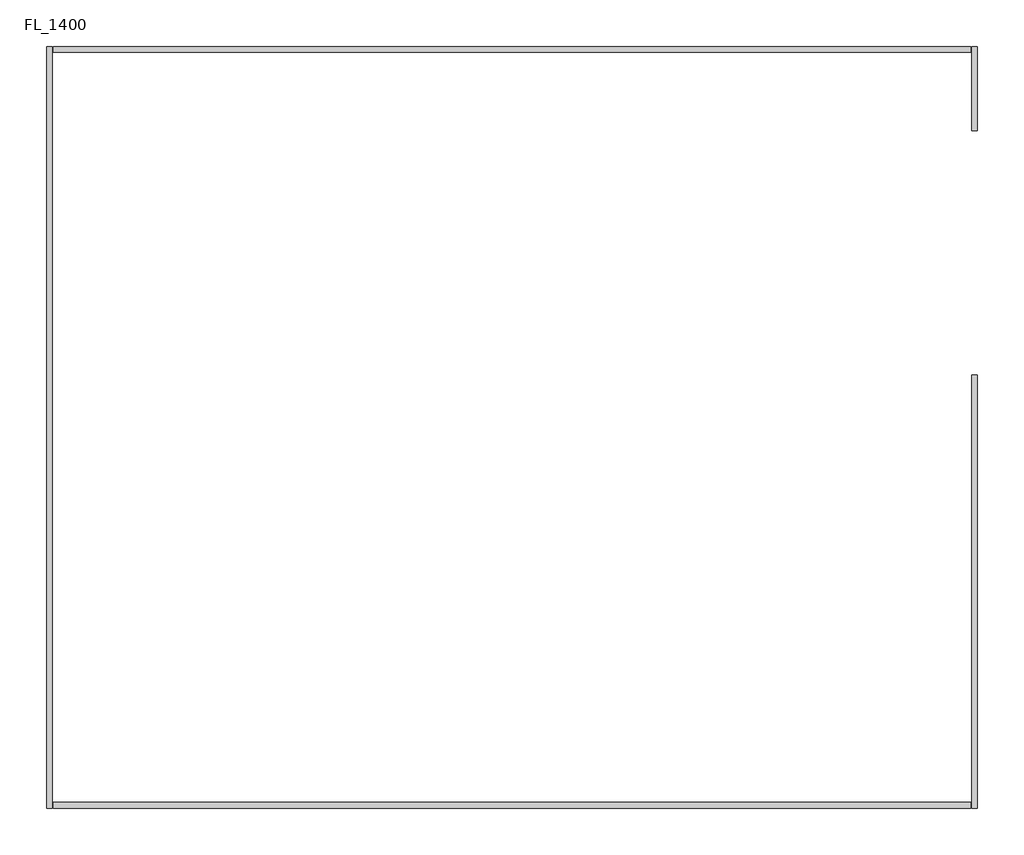
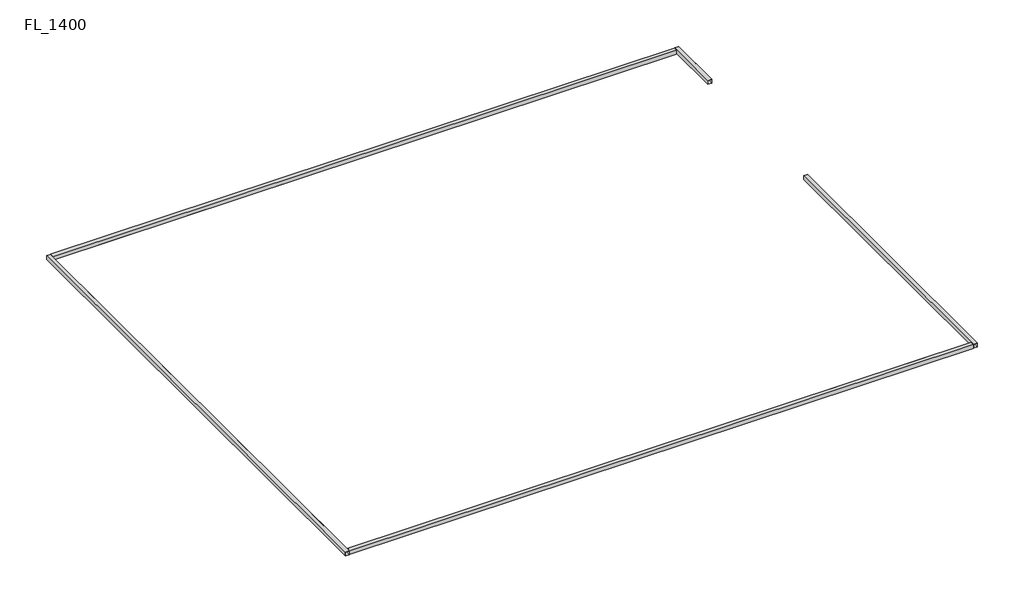
# One storey: 5 beams.
"""IFC4 building model written with IfcOpenShell, lengths in millimetres."""

import ifcopenshell
import ifcopenshell.guid

model = None  # the IFC model being written
_history = None  # IfcOwnerHistory: only IFC2X3 demands one
_inside = {}  # id of a spatial element -> (the spatial element, [elements in it])
_under = {}  # id of a project, library or spatial element -> (it, [spatial elements below it])
_declared = {}  # id of a project -> (the project, [libraries it declares])
_typed = {}  # id of a type object -> (the type object, [elements of that type])
_made_of = {}  # id of a material, layer set ... -> (it, [elements and type objects made of it])


def new_model(schema):
    """Start an empty IFC model of exactly this schema.

    Asked for "IFC4X3", IfcOpenShell would pick the latest addendum, in which some entities
    have other attributes; the version numbers below select the first issue.
    IFC2X3 requires an IfcOwnerHistory on every rooted entity: one is made here for all.
    """
    global model, _history
    if schema == "IFC4X3":
        model = ifcopenshell.file(schema_version=(4, 3, 0, 0))
    else:
        model = ifcopenshell.file(schema=schema)
    _inside.clear()
    _under.clear()
    _declared.clear()
    _typed.clear()
    _made_of.clear()
    _history = None
    if model.schema == "IFC2X3":
        org = make("IfcOrganization", Name="unknown")
        user = make(
            "IfcPersonAndOrganization",
            ThePerson=make("IfcPerson", FamilyName="unknown"),
            TheOrganization=org,
        )
        app = make(
            "IfcApplication",
            ApplicationDeveloper=org,
            Version="unknown",
            ApplicationFullName="unknown",
            ApplicationIdentifier="unknown",
        )
        _history = make(
            "IfcOwnerHistory",
            OwningUser=user,
            OwningApplication=app,
            ChangeAction="ADDED",
            CreationDate=0,
        )
    return model


def make(cls, **values):
    """One entity of the class cls with the attributes given. An attribute that is None is left unset."""
    return model.create_entity(
        cls, **{name: value for name, value in values.items() if value is not None}
    )


def rooted(cls, **values):
    """An entity with a GlobalId (a new one), such as an element, a storey or a relation."""
    return make(cls, GlobalId=ifcopenshell.guid.new(), OwnerHistory=_history, **values)


def si_unit(unit_type, name, prefix=None):
    """IfcSIUnit, for example si_unit("LENGTHUNIT", "METRE", prefix="MILLI")."""
    return make("IfcSIUnit", UnitType=unit_type, Prefix=prefix, Name=name)


def assignment(units):
    """IfcUnitAssignment: the units of a project."""
    return None if units is None else make("IfcUnitAssignment", Units=units)


def point(xyz):
    """IfcCartesianPoint."""
    return None if xyz is None else make("IfcCartesianPoint", Coordinates=xyz)


def direction(xyz):
    """IfcDirection."""
    return None if xyz is None else make("IfcDirection", DirectionRatios=xyz)


def frame(location, z_axis=None, x_axis=None):
    """IfcAxis2Placement3D, a coordinate frame: its origin and axes. An axis left out is left unset."""
    return make(
        "IfcAxis2Placement3D",
        Location=point(location),
        Axis=direction(z_axis),
        RefDirection=direction(x_axis),
    )


def origin():
    """The frame at (0, 0, 0) with its axes left unset."""
    return frame((0.0, 0.0, 0.0))


def place(relative_to, where):
    """IfcLocalPlacement: puts the frame where relative to a parent placement (None: the world)."""
    return make(
        "IfcLocalPlacement", PlacementRelTo=relative_to, RelativePlacement=where
    )


def context(
    kind, dimensions, precision=None, world=None, true_north=None, identifier=None
):
    """IfcGeometricRepresentationContext, for example the 3D "Model" context."""
    return make(
        "IfcGeometricRepresentationContext",
        ContextIdentifier=identifier,
        ContextType=kind,
        CoordinateSpaceDimension=dimensions,
        Precision=precision,
        WorldCoordinateSystem=world,
        TrueNorth=true_north,
    )


def project(units=None, contexts=None):
    """IfcProject with its units and contexts."""
    return rooted(
        "IfcProject",
        Name="project",
        RepresentationContexts=contexts,
        UnitsInContext=assignment(units),
    )


def spatial(cls, under=None, at=None, **own):
    """A site, building, storey or space (cls), placed at a placement, below another one or the project."""
    s = rooted(cls, ObjectPlacement=at, **own)
    if under is not None:
        _under.setdefault(under.id(), (under, []))[1].append(s)
    return s


def polyline(points):
    """IfcPolyline through the points."""
    return make("IfcPolyline", Points=[point(p) for p in points])


def outline(outer, holes=None, kind="AREA"):
    """IfcArbitraryClosedProfileDef: a profile drawn as a closed curve; with holes, ...WithVoids."""
    if holes is None:
        return make("IfcArbitraryClosedProfileDef", ProfileType=kind, OuterCurve=outer)
    return make(
        "IfcArbitraryProfileDefWithVoids",
        ProfileType=kind,
        OuterCurve=outer,
        InnerCurves=holes,
    )


def extrude(swept, where, along, depth):
    """IfcExtrudedAreaSolid: the profile swept, set in the frame where, extruded along a direction by depth."""
    return make(
        "IfcExtrudedAreaSolid",
        SweptArea=swept,
        Position=where,
        ExtrudedDirection=direction(along),
        Depth=depth,
    )


def shape(context_of_items, identifier, shape_type, items):
    """IfcShapeRepresentation: the items that make up one representation, for example the "Body"."""
    return make(
        "IfcShapeRepresentation",
        ContextOfItems=context_of_items,
        RepresentationIdentifier=identifier,
        RepresentationType=shape_type,
        Items=items,
    )


def source(mapping_origin, context_of_items, identifier, shape_type, items):
    """IfcRepresentationMap: a shape defined once, which mapped items show again and again."""
    return make(
        "IfcRepresentationMap",
        MappingOrigin=mapping_origin,
        MappedRepresentation=shape(context_of_items, identifier, shape_type, items),
    )


def transform(
    local_origin,
    x_axis=None,
    y_axis=None,
    z_axis=None,
    scale=None,
    scale2=None,
    scale3=None,
    uniform=True,
):
    """IfcCartesianTransformationOperator3D, or its non-uniform kind. x_axis, y_axis, z_axis: its Axis1, 2, 3."""
    if uniform:
        return make(
            "IfcCartesianTransformationOperator3D",
            Axis1=direction(x_axis),
            Axis2=direction(y_axis),
            LocalOrigin=point(local_origin),
            Scale=scale,
            Axis3=direction(z_axis),
        )
    return make(
        "IfcCartesianTransformationOperator3DnonUniform",
        Axis1=direction(x_axis),
        Axis2=direction(y_axis),
        LocalOrigin=point(local_origin),
        Scale=scale,
        Axis3=direction(z_axis),
        Scale2=scale2,
        Scale3=scale3,
    )


def mapped(mapping_source, mapping_target):
    """IfcMappedItem: shows the shape of a source again, moved by a transform."""
    return make(
        "IfcMappedItem", MappingSource=mapping_source, MappingTarget=mapping_target
    )


def made_of(thing, what):
    """Note that an element or type object is made of a material, layer set ...; save() writes the relation."""
    if what is not None:
        _made_of.setdefault(what.id(), (what, []))[1].append(thing)
    return thing


def element(
    cls,
    number,
    at=None,
    inside=None,
    cuts=None,
    type_object=None,
    material=None,
    context=None,
    identifier="Body",
    shape_type=None,
    held_by="IfcProductDefinitionShape",
    body=None,
    shapes=None,
    **own,
):
    """One element of the class cls, such as IfcWall. Its Tag is "e" and its number.

    at: its placement. inside: the storey or other place that contains it. cuts: it is an
    opening in that element (IfcRelVoidsElement). A single representation is given by context,
    identifier, shape_type and body (its items); several are given by shapes. held_by: the class
    of the entity that holds the representations. save() writes the other relations.
    """
    e = rooted(cls, Tag="e%d" % number, ObjectPlacement=at, **own)
    if body is not None:
        shapes = [shape(context, identifier, shape_type, body)]
    if shapes is not None:
        e.Representation = make(held_by, Representations=shapes)
    if inside is not None:
        _inside.setdefault(inside.id(), (inside, []))[1].append(e)
    if cuts is not None:
        rooted(
            "IfcRelVoidsElement", RelatingBuildingElement=cuts, RelatedOpeningElement=e
        )
    if type_object is not None:
        _typed.setdefault(type_object.id(), (type_object, []))[1].append(e)
    return made_of(e, material)


def aggregate(whole, parts):
    """IfcRelAggregates: a whole, such as a stair, and the parts it consists of."""
    return rooted("IfcRelAggregates", RelatingObject=whole, RelatedObjects=parts)


def save(model, path):
    """Write the relations noted so far, then the file.

    IfcRelAggregates (storeys below a building ...), IfcRelContainedInSpatialStructure (elements
    in a storey), IfcRelDefinesByType, IfcRelAssociatesMaterial and IfcRelDeclares: one each for
    every whole, place, type object, material and project.
    """
    for whole, parts in _under.values():
        aggregate(whole, parts)
    for where, things in _inside.values():
        rooted(
            "IfcRelContainedInSpatialStructure",
            RelatedElements=things,
            RelatingStructure=where,
        )
    for kind, things in _typed.values():
        rooted("IfcRelDefinesByType", RelatedObjects=things, RelatingType=kind)
    for what, things in _made_of.values():
        rooted("IfcRelAssociatesMaterial", RelatedObjects=things, RelatingMaterial=what)
    for by, libraries in _declared.values():
        rooted("IfcRelDeclares", RelatingContext=by, RelatedDefinitions=libraries)
    model.write(path)


def steel_rectangular_beam_bm125_rt_100x100x4_0_fd47acba(model_context):
    return source(origin(), model_context, "Body", "SweptSolid", [
        extrude(outline(polyline([(-50.0, 50.0), (50.0, 50.0), (50.0, -50.0), (-50.0, -50.0), (-50.0, 50.0)]), holes=[polyline([(46.0, -46.0), (46.0, 46.0), (-46.0, 46.0), (-46.0, -46.0), (46.0, -46.0)])]), frame((-7887.3, 0.0, 0.0), z_axis=(1.0, 0.0, 0.0), x_axis=(0.0, 1.0, 0.0)), (0.0, 0.0, 1.0), 15774.6),
        extrude(outline(polyline([(-50.0, 50.0), (50.0, 50.0), (50.0, -50.0), (-50.0, -50.0), (-50.0, 50.0)]), holes=[polyline([(46.0, -46.0), (46.0, 46.0), (-46.0, 46.0), (-46.0, -46.0), (46.0, -46.0)])]), frame((-7887.3, 0.0, 0.0), z_axis=(1.0, 0.0, 0.0), x_axis=(0.0, 1.0, 0.0)), (0.0, 0.0, 1.0), 15774.6),
        extrude(outline(polyline([(-50.0, 50.0), (50.0, 50.0), (50.0, -50.0), (-50.0, -50.0), (-50.0, 50.0)]), holes=[polyline([(46.0, -46.0), (46.0, 46.0), (-46.0, 46.0), (-46.0, -46.0), (46.0, -46.0)])]), frame((-7887.3, 0.0, 0.0), z_axis=(1.0, 0.0, 0.0), x_axis=(0.0, 1.0, 0.0)), (0.0, 0.0, 1.0), 15774.6),
        extrude(outline(polyline([(-50.0, 50.0), (50.0, 50.0), (50.0, -50.0), (-50.0, -50.0), (-50.0, 50.0)]), holes=[polyline([(46.0, -46.0), (46.0, 46.0), (-46.0, 46.0), (-46.0, -46.0), (46.0, -46.0)])]), frame((-7887.3, 0.0, 0.0), z_axis=(1.0, 0.0, 0.0), x_axis=(0.0, 1.0, 0.0)), (0.0, 0.0, 1.0), 15774.6),
    ])


def steel_rectangular_beam_bm125_rt_100x100x4_0_2c93a6f0(model_context):
    return source(origin(), model_context, "Body", "SweptSolid", [
        extrude(outline(polyline([(-50.0, 50.0), (50.0, 50.0), (50.0, -50.0), (-50.0, -50.0), (-50.0, 50.0)]), holes=[polyline([(46.0, -46.0), (46.0, 46.0), (-46.0, 46.0), (-46.0, -46.0), (46.0, -46.0)])]), frame((-6550.0, 0.0, 0.0), z_axis=(1.0, 0.0, 0.0), x_axis=(0.0, 1.0, 0.0)), (0.0, 0.0, 1.0), 13100.0),
        extrude(outline(polyline([(-50.0, 50.0), (50.0, 50.0), (50.0, -50.0), (-50.0, -50.0), (-50.0, 50.0)]), holes=[polyline([(46.0, -46.0), (46.0, 46.0), (-46.0, 46.0), (-46.0, -46.0), (46.0, -46.0)])]), frame((-6550.0, 0.0, 0.0), z_axis=(1.0, 0.0, 0.0), x_axis=(0.0, 1.0, 0.0)), (0.0, 0.0, 1.0), 13100.0),
        extrude(outline(polyline([(-50.0, 50.0), (50.0, 50.0), (50.0, -50.0), (-50.0, -50.0), (-50.0, 50.0)]), holes=[polyline([(46.0, -46.0), (46.0, 46.0), (-46.0, 46.0), (-46.0, -46.0), (46.0, -46.0)])]), frame((-6550.0, 0.0, 0.0), z_axis=(1.0, 0.0, 0.0), x_axis=(0.0, 1.0, 0.0)), (0.0, 0.0, 1.0), 13100.0),
        extrude(outline(polyline([(-50.0, 50.0), (50.0, 50.0), (50.0, -50.0), (-50.0, -50.0), (-50.0, 50.0)]), holes=[polyline([(46.0, -46.0), (46.0, 46.0), (-46.0, 46.0), (-46.0, -46.0), (46.0, -46.0)])]), frame((-6550.0, 0.0, 0.0), z_axis=(1.0, 0.0, 0.0), x_axis=(0.0, 1.0, 0.0)), (0.0, 0.0, 1.0), 13100.0),
    ])


def steel_rectangular_beam_bm125_rt_100x100x4_0_60a5dd41(model_context):
    return source(origin(), model_context, "Body", "SweptSolid", [
        extrude(outline(polyline([(-50.0, 50.0), (50.0, 50.0), (50.0, -50.0), (-50.0, -50.0), (-50.0, 50.0)]), holes=[polyline([(46.0, -46.0), (46.0, 46.0), (-46.0, 46.0), (-46.0, -46.0), (46.0, -46.0)])]), frame((-3725.0, 0.0, 0.0), z_axis=(1.0, 0.0, 0.0), x_axis=(0.0, 1.0, 0.0)), (0.0, 0.0, 1.0), 7450.0),
        extrude(outline(polyline([(-50.0, 50.0), (50.0, 50.0), (50.0, -50.0), (-50.0, -50.0), (-50.0, 50.0)]), holes=[polyline([(46.0, -46.0), (46.0, 46.0), (-46.0, 46.0), (-46.0, -46.0), (46.0, -46.0)])]), frame((-3725.0, 0.0, 0.0), z_axis=(1.0, 0.0, 0.0), x_axis=(0.0, 1.0, 0.0)), (0.0, 0.0, 1.0), 7450.0),
        extrude(outline(polyline([(-50.0, 50.0), (50.0, 50.0), (50.0, -50.0), (-50.0, -50.0), (-50.0, 50.0)]), holes=[polyline([(46.0, -46.0), (46.0, 46.0), (-46.0, 46.0), (-46.0, -46.0), (46.0, -46.0)])]), frame((-3725.0, 0.0, 0.0), z_axis=(1.0, 0.0, 0.0), x_axis=(0.0, 1.0, 0.0)), (0.0, 0.0, 1.0), 7450.0),
        extrude(outline(polyline([(-50.0, 50.0), (50.0, 50.0), (50.0, -50.0), (-50.0, -50.0), (-50.0, 50.0)]), holes=[polyline([(46.0, -46.0), (46.0, 46.0), (-46.0, 46.0), (-46.0, -46.0), (46.0, -46.0)])]), frame((-3725.0, 0.0, 0.0), z_axis=(1.0, 0.0, 0.0), x_axis=(0.0, 1.0, 0.0)), (0.0, 0.0, 1.0), 7450.0),
    ])


def steel_rectangular_beam_bm125_rt_100x100x4_0_366960fc(model_context):
    return source(origin(), model_context, "Body", "SweptSolid", [
        extrude(outline(polyline([(-50.0, 50.0), (50.0, 50.0), (50.0, -50.0), (-50.0, -50.0), (-50.0, 50.0)]), holes=[polyline([(46.0, -46.0), (46.0, 46.0), (-46.0, 46.0), (-46.0, -46.0), (46.0, -46.0)])]), frame((-725.0, 0.0, 0.0), z_axis=(1.0, 0.0, 0.0), x_axis=(0.0, 1.0, 0.0)), (0.0, 0.0, 1.0), 1450.0),
        extrude(outline(polyline([(-50.0, 50.0), (50.0, 50.0), (50.0, -50.0), (-50.0, -50.0), (-50.0, 50.0)]), holes=[polyline([(46.0, -46.0), (46.0, 46.0), (-46.0, 46.0), (-46.0, -46.0), (46.0, -46.0)])]), frame((-725.0, 0.0, 0.0), z_axis=(1.0, 0.0, 0.0), x_axis=(0.0, 1.0, 0.0)), (0.0, 0.0, 1.0), 1450.0),
        extrude(outline(polyline([(-50.0, 50.0), (50.0, 50.0), (50.0, -50.0), (-50.0, -50.0), (-50.0, 50.0)]), holes=[polyline([(46.0, -46.0), (46.0, 46.0), (-46.0, 46.0), (-46.0, -46.0), (46.0, -46.0)])]), frame((-725.0, 0.0, 0.0), z_axis=(1.0, 0.0, 0.0), x_axis=(0.0, 1.0, 0.0)), (0.0, 0.0, 1.0), 1450.0),
        extrude(outline(polyline([(-50.0, 50.0), (50.0, 50.0), (50.0, -50.0), (-50.0, -50.0), (-50.0, 50.0)]), holes=[polyline([(46.0, -46.0), (46.0, 46.0), (-46.0, 46.0), (-46.0, -46.0), (46.0, -46.0)])]), frame((-725.0, 0.0, 0.0), z_axis=(1.0, 0.0, 0.0), x_axis=(0.0, 1.0, 0.0)), (0.0, 0.0, 1.0), 1450.0),
    ])


model = new_model("IFC4")

# Units and contexts
model_context = context("Model", 3, world=origin())
ifc_project = project(units=[si_unit("LENGTHUNIT", "METRE", prefix="MILLI")], contexts=[model_context])

# Site, building, storey
site = spatial("IfcSite", under=ifc_project)
building = spatial("IfcBuilding", under=site)
storey = spatial("IfcBuildingStorey", under=building, Name="FL_1400", Elevation=1400.0)

# Beams
placement = place(None, origin())
steel_rectangular_beam_bm125_rt_100x100x4_0_shape = steel_rectangular_beam_bm125_rt_100x100x4_0_fd47acba(model_context)
element("IfcBeam", 1, ObjectType="Steel-Rectangular-Beam : BM125_RT-100x100x4.0", at=placement, inside=storey, context=model_context, shape_type="MappedRepresentation", body=[
    mapped(steel_rectangular_beam_bm125_rt_100x100x4_0_shape, transform((6100.0, 10094.5382614, 1350.0), x_axis=(1.0, 0.0, 0.0), y_axis=(0.0, 1.0, 0.0), z_axis=(0.0, 0.0, 1.0))),
])
element("IfcBeam", 2, ObjectType="Steel-Rectangular-Beam : BM125_RT-100x100x4.0", at=placement, inside=storey, context=model_context, shape_type="MappedRepresentation", body=[
    mapped(steel_rectangular_beam_bm125_rt_100x100x4_0_shape, transform((6100.0, 23094.5382614, 1350.0), x_axis=(-1.0, 0.0, 0.0), y_axis=(0.0, -1.0, 0.0), z_axis=(0.0, 0.0, 1.0))),
])
steel_rectangular_beam_bm125_rt_100x100x4_0_2_shape = steel_rectangular_beam_bm125_rt_100x100x4_0_2c93a6f0(model_context)
element("IfcBeam", 3, ObjectType="Steel-Rectangular-Beam : BM125_RT-100x100x4.0", at=placement, inside=storey, context=model_context, shape_type="MappedRepresentation", body=[
    mapped(steel_rectangular_beam_bm125_rt_100x100x4_0_2_shape, transform((-1850.0, 16594.5382614, 1350.0), x_axis=(0.0, -1.0, 0.0), y_axis=(1.0, 0.0, 0.0), z_axis=(0.0, 0.0, 1.0))),
])
steel_rectangular_beam_bm125_rt_100x100x4_0_3_shape = steel_rectangular_beam_bm125_rt_100x100x4_0_60a5dd41(model_context)
element("IfcBeam", 4, ObjectType="Steel-Rectangular-Beam : BM125_RT-100x100x4.0", at=placement, inside=storey, context=model_context, shape_type="MappedRepresentation", body=[
    mapped(steel_rectangular_beam_bm125_rt_100x100x4_0_3_shape, transform((14050.0, 13769.5382614, 1350.0), x_axis=(0.0, 1.0, 0.0), y_axis=(-1.0, 0.0, 0.0), z_axis=(0.0, 0.0, 1.0))),
])
steel_rectangular_beam_bm125_rt_100x100x4_0_4_shape = steel_rectangular_beam_bm125_rt_100x100x4_0_366960fc(model_context)
element("IfcBeam", 5, ObjectType="Steel-Rectangular-Beam : BM125_RT-100x100x4.0", at=placement, inside=storey, context=model_context, shape_type="MappedRepresentation", body=[
    mapped(steel_rectangular_beam_bm125_rt_100x100x4_0_4_shape, transform((14050.0, 22419.5382614, 1350.0), x_axis=(0.0, 1.0, 0.0), y_axis=(-1.0, 0.0, 0.0), z_axis=(0.0, 0.0, 1.0))),
])

save(model, "model.ifc")

# Revit data of these elements
# Type "Steel-Rectangular-Beam : BM125_RT-100x100x4.0"
#   t = 4 mm
#   Mass per Unit Length = 11.70 kg/m
#   Surface Area = 0.386 m²/m
#   Sectional Area = 14.95 cm²
#   Length [instance default] = 3000 mm
#   H = 100 mm
#   B = 100 mm
#   hec_material4 [instance default] = none
#   hec_material3 [instance default] = none
#   hec_material2 [instance default] = none
#   hec_material1 [instance default] = none
#   Structural Material [instance default] = none
# Elements 1, 2, 3, 4, 5 (IfcBeam, "Steel-Rectangular-Beam : BM125_RT-100x100x4.0")
#   Comments = ""
#   F01) Building Name = "Fire Water Pump Building"
#   F11) Project Building Tag_Type-1 = ""
#   F12) Project Building Tag_Type-2 = ""
#   F13) Project Facility Code = "621"
#   F21) Structural Type = "Steel"
#   F31) Standard Building Code = "E204"
#   F41) Discipline = "Architecture"
#   F51) Plan Start Date-Engineering = "2018-09-14"
#   F52) Plan Finish Date-Engineering = "2019-12-02"
#   F53) Duration = "444"
#   W11) Activity ID = "T3C621AR4110"
#   W12) Activity Name = "Fire Water Pump BLDG - Main Steel Structure"
#   W13) Plan Start Date = "2019-04-02"
#   W14) Plan Finish Date = "2019-06-03"
#   hec_material4 = none
#   hec_material3 = none
#   hec_material2 = S01AA010-00001_Main Steel Structure Fabrication Work_Shelter/Building_Steel Painting/Coating_for Non-Fireproofed Steel Surface, Surface Preparation, Primer, Second & Final Coat
#   hec_material1 = S03AA007-00001_Main Steel Structure Erection Work_Girth & Purlin
#   Structural Material = S01AA007-00001_Main Steel Structure Fabrication Work_Shelter/Building_Girth & Purlin
#   Phase Created = New Construction
#   Materials on its faces: "S01AA010-00001_Main Steel Structure Fabrication Work_Shelter/Building_Steel Painting/Coating_for Non-Fireproofed Steel Surface, Surface Preparation, Primer, Second & Final Coat"
# Materials
#   "S01AA010-00001_Main Steel Structure Fabrication Work_Shelter/Building_Steel Painting/Coating_for Non-Fireproofed Steel Surface, Surface Preparation, Primer, Second & Final Coat": class "Metal", colour RGB 120 120 120, transparency 0, Description = "Paint finished steel", W00) Work Master Code = "S01AA010-00001", W01) Work Master_Lv1 = "Main Steel Structure Fabrication Work", W02) Work Master_Lv2 = "Shelter/Building", W03) Work Master_Spec.1 = "Steel Painting/Coating", W04) Work Master_Spec.2 = "for Non-Fireproofed Steel Surface, Surface Preparation, Primer, Second & Final Coat", Cost = 0
#   "S03AA007-00001_Main Steel Structure Erection Work_Girth & Purlin": class "Metal", colour RGB 120 120 120, transparency 0, Comments = "(30KG/M>Weight)", Description = "Structural steel 50ksi", W00) Work Master Code = "S03AA007-00001", W01) Work Master_Lv1 = "Main Steel Structure Erection Work", W02) Work Master_Lv2 = "Shelter/Building", W03) Work Master_Spec.1 = "Girth & Purlin", Cost = 0
#   "S01AA007-00001_Main Steel Structure Fabrication Work_Shelter/Building_Girth & Purlin": class "Metal", colour RGB 120 120 120, transparency 0, Comments = "(30KG/M>Weight)", Description = "Structural steel 50ksi", W00) Work Master Code = "S01AA007-00001", W01) Work Master_Lv1 = "Main Steel Structure Fabrication Work", W02) Work Master_Lv2 = "Shelter/Building", W03) Work Master_Spec.1 = "Girth & Purlin", Cost = 0
